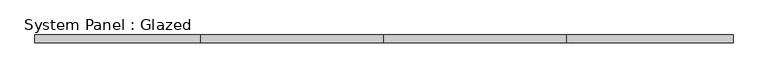
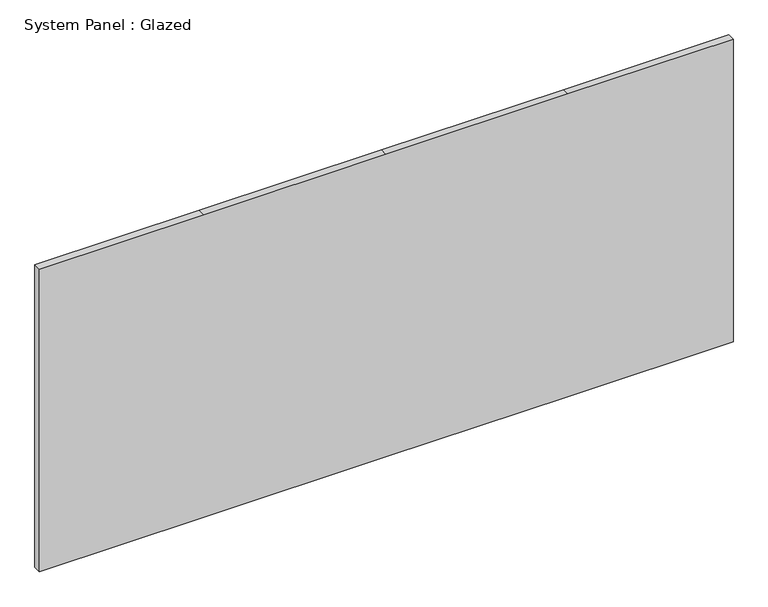
"""IFC4 building model written with IfcOpenShell, lengths in millimetres: plate geometry, System Panel : Glazed."""

from ifc_helpers import new_model, si_unit, frame, origin, place, context, project, spatial, polyline, outline, extrude, source, transform, mapped, element, save


def system_panel_glazed_6cd02bc8(model_context):
    return source(origin(), model_context, "Body", "SweptSolid", [
        extrude(outline(polyline([(0.0, -2286.9812356), (0.0, -1202.0187644), (0.0, -2.0187644), (0.0, 1197.9812356), (0.0, 2286.9812356), (2110.0, 2286.9812356), (2110.0, 1197.9812356), (2110.0, -2.0187644), (2110.0, -1202.0187644), (2110.0, -2286.9812356), (0.0, -2286.9812356)])), frame((0.0, -25.0, 0.0), z_axis=(0.0, 1.0, 0.0), x_axis=(0.0, 0.0, 1.0)), (0.0, 0.0, 1.0), 50.0),
    ])


if __name__ == "__main__":
    model = new_model("IFC4")
    model_context = context("Model", 3, world=origin())
    ifc_project = project(units=[si_unit("LENGTHUNIT", "METRE", prefix="MILLI")], contexts=[model_context])
    site = spatial("IfcSite", under=ifc_project)
    building = spatial("IfcBuilding", under=site)
    placement = place(None, origin())
    system_panel_glazed_shape = system_panel_glazed_6cd02bc8(model_context)
    element("IfcPlate", 1, ObjectType="System Panel : Glazed", at=placement, inside=building, context=model_context, shape_type="MappedRepresentation", body=[
        mapped(system_panel_glazed_shape, transform((0.0, 0.0, 0.0), x_axis=(1.0, 0.0, 0.0), y_axis=(0.0, 1.0, 0.0), z_axis=(0.0, 0.0, 1.0))),
    ])
    save(model, "model.ifc")

# Revit data of these elements
# Type "System Panel : Glazed"
#   Type Mark = "CW-GLASS"
# Element 1 (IfcPlate, "System Panel : Glazed")
#   Materials on its faces: "Glass_Clear"
# Materials
#   "Glass_Clear": class "Glass", colour RGB 128 128 255, transparency 0.8, Comments = "Rendering appearance not upgraded ", Cost = 0
